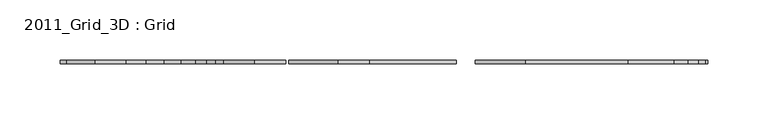
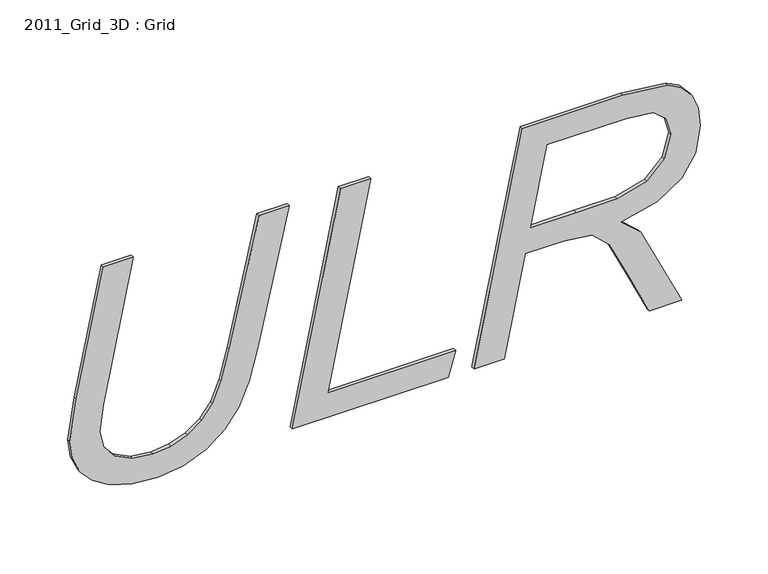
"""IFC4 building model written with IfcOpenShell, lengths in millimetres: proxy geometry, 2011_Grid_3D : Grid."""

from ifc_helpers import new_model, si_unit, frame, origin, place, context, project, spatial, polyline, outline, extrude, source, transform, mapped, element, save


def proxy_2011_grid_3d_grid_3cac8b31(model_context):
    return source(origin(), model_context, "Body", "SweptSolid", [
        extrude(outline(polyline([(101.4447294, 32343.9093434), (-9.5457855, 32320.8090397), (-46.3278141, 32315.1578924), (-62.2836301, 32317.3018584), (-76.4424804, 32323.7337562), (-88.2714718, 32334.4659789), (-97.2377109, 32349.5109192), (-102.8888581, 32368.2985052), (-104.7725739, 32390.2586651), (-102.1081075, 32412.4542896), (-94.1147085, 32431.7499831), (-81.7032524, 32447.6500312), (-65.784615, 32459.6587191), (-44.9584024, 32468.7550833), (-17.8242205, 32475.9181603), (101.4447294, 32503.0833243), (101.4447294, 32477.157447), (-10.7355007, 32451.57857), (-36.7791103, 32444.8864219), (-54.6310349, 32437.4011304), (-66.7202764, 32428.1064803), (-75.4758368, 32415.9862566), (-80.7923767, 32401.9079599), (-82.5645566, 32386.739091), (-80.0983761, 32368.639309), (-72.6998347, 32353.897994), (-61.2488258, 32344.1014328), (-46.6252429, 32340.8359124), (-23.5745107, 32343.9589148), (101.4447294, 32369.6369348), (101.4447294, 32343.9093434)])), frame((0.0, -3.175, 0.0), z_axis=(0.0, 1.0, 0.0), x_axis=(0.0, 0.0, 1.0)), (0.0, 0.0, 1.0), 3.175),
        extrude(outline(polyline([(-101.6, 32505.5123262), (-101.6, 32638.7604299), (-79.3919827, 32645.1055777), (-79.3919827, 32535.8004926), (101.4447294, 32572.5329498), (101.4447294, 32546.7557869), (-101.6, 32505.5123262)])), frame((0.0, -3.175, 0.0), z_axis=(0.0, 1.0, 0.0), x_axis=(0.0, 0.0, 1.0)), (0.0, 0.0, 1.0), 3.175),
        extrude(outline(polyline([(-101.6, 32660.9684472), (-101.6, 32686.7456101), (-12.7679309, 32704.7896241), (-12.7679309, 32737.6555068), (-15.9652905, 32762.0198829), (-29.4239439, 32776.4203941), (-64.4213996, 32793.1259785), (-101.6, 32810.8725638), (-101.6, 32838.5830139), (-64.6196855, 32820.9355716), (-27.4906566, 32803.2385578), (-12.7679309, 32786.5329734), (-4.8736748, 32817.4283903), (8.8948002, 32838.4342995), (27.7567435, 32850.480166), (50.9314044, 32854.4954548), (67.4758815, 32852.6303284), (80.922142, 32847.034949), (90.9231855, 32838.1616564), (97.1320117, 32826.4627902), (101.4447294, 32787.970546), (101.4447294, 32702.2119078), (-101.6, 32660.9684472)]), holes=[polyline([(9.4400864, 32709.3006276), (79.2367121, 32723.4780672), (79.2367121, 32791.4405487), (76.8077102, 32814.1938521), (67.6122031, 32825.0004319), (51.7245478, 32829.1148637), (31.524175, 32823.7115738), (16.5783776, 32808.5179191), (9.4400864, 32783.3603995), (9.4400864, 32748.2142293), (9.4400864, 32709.3006276)])]), frame((0.0, -3.175, 0.0), z_axis=(0.0, 1.0, 0.0), x_axis=(0.0, 0.0, 1.0)), (0.0, 0.0, 1.0), 3.175),
    ])


if __name__ == "__main__":
    model = new_model("IFC4")
    model_context = context("Model", 3, world=origin())
    ifc_project = project(units=[si_unit("LENGTHUNIT", "METRE", prefix="MILLI")], contexts=[model_context])
    site = spatial("IfcSite", under=ifc_project)
    building = spatial("IfcBuilding", under=site)
    placement = place(None, origin())
    proxy_2011_grid_3d_grid_shape = proxy_2011_grid_3d_grid_3cac8b31(model_context)
    element("IfcBuildingElementProxy", 1, Name="2011_Grid_3D : Grid", ObjectType="2011_Grid_3D : Grid", at=placement, inside=building, context=model_context, shape_type="MappedRepresentation", body=[
        mapped(proxy_2011_grid_3d_grid_shape, transform((0.0, 0.0, 0.0), x_axis=(1.0, 0.0, 0.0), y_axis=(0.0, 1.0, 0.0), z_axis=(0.0, 0.0, 1.0))),
    ])
    save(model, "model.ifc")

# Revit data of these elements
# Type "2011_Grid_3D : Grid"
#   Workplane [instance default] = "LEVEL"
#   Grid [instance default] = "S"
#   t [instance default] = 12' - 6"
#   built-in parameter 1001306 [instance default] = 50 (stored number, unit not read)
#   d [instance default] = 2
#   Symbol At End 2 [instance default] = yes
#   Symbol At End 1 [instance default] = yes
#   Robust [instance default] = yes
#   No of grid markers [instance default] = 3
#   Grid Height Visible = yes
#   Height = 0
#   Assembly Code = ""
# Element 1 (IfcBuildingElementProxy, "2011_Grid_3D : Grid")
#   Workplane = "ULR"
#   Grid = "1"
#   t = 13' - 2.15638"
#   built-in parameter 1001306 = 105.438 (stored number, unit not read)
#   d = 4
#   Robust = no
#   No of grid markers = 5
#   Materials on its faces: "Letter"
# Materials
#   "Letter": class "Unassigned", colour RGB 178 187 30, transparency 0, Comments = "Rendering appearance not upgraded "
